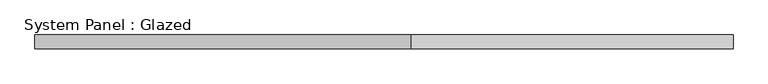
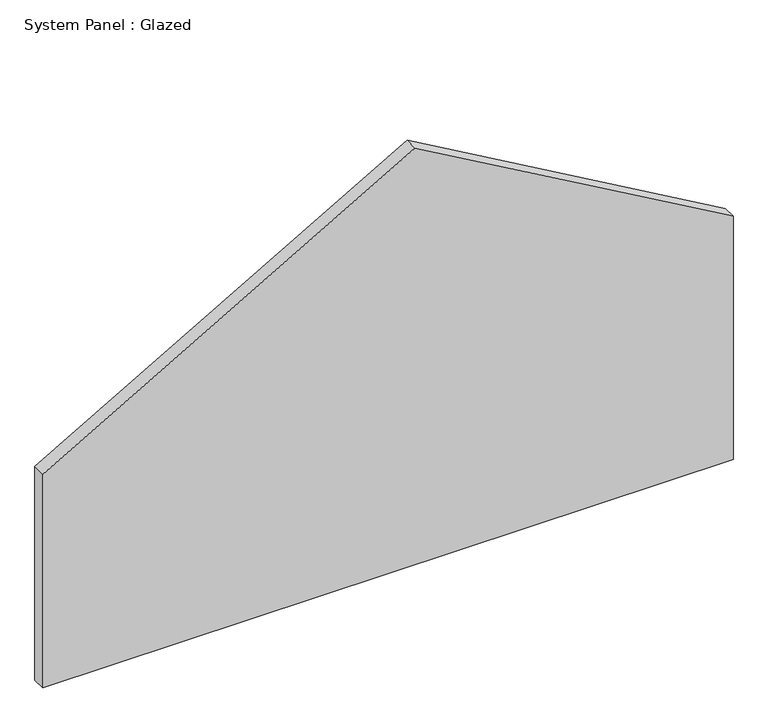
"""IFC4 building model written with IfcOpenShell, lengths in millimetres: plate geometry, System Panel : Glazed."""

from ifc_helpers import new_model, si_unit, frame, origin, place, context, project, spatial, polyline, outline, extrude, source, transform, mapped, element, save


def system_panel_glazed_71429794(model_context):
    return source(origin(), model_context, "Body", "SweptSolid", [
        extrude(outline(polyline([(0.0, -639.2857142), (0.0, 639.2857142), (476.2276186, 639.2857142), (816.4518843, 50.0), (418.4925917, -639.2857142), (0.0, -639.2857142)])), frame((0.0, 24.5, 0.0), z_axis=(0.0, 1.0, 0.0), x_axis=(0.0, 0.0, 1.0)), (0.0, 0.0, 1.0), 25.0),
    ])


if __name__ == "__main__":
    model = new_model("IFC4")
    model_context = context("Model", 3, world=origin())
    ifc_project = project(units=[si_unit("LENGTHUNIT", "METRE", prefix="MILLI")], contexts=[model_context])
    site = spatial("IfcSite", under=ifc_project)
    building = spatial("IfcBuilding", under=site)
    placement = place(None, origin())
    system_panel_glazed_shape = system_panel_glazed_71429794(model_context)
    element("IfcPlate", 1, ObjectType="System Panel : Glazed", at=placement, inside=building, context=model_context, shape_type="MappedRepresentation", body=[
        mapped(system_panel_glazed_shape, transform((0.0, 0.0, 0.0), x_axis=(1.0, 0.0, 0.0), y_axis=(0.0, 1.0, 0.0), z_axis=(0.0, 0.0, 1.0))),
    ])
    save(model, "model.ifc")

# Revit data of these elements
# Type "System Panel : Glazed"
#   Construction Type Id = "GSP4R"
#   Analytic Construction = "1/8 in Pilkington single glazing"
#   Visual Light Transmittance = 0.9
#   Solar Heat Gain Coefficient = 0.86
#   Heat Transfer Coefficient (U) = 6.7069 W/(m²·K)
#   Define Thermal Properties by = 1
# Element 1 (IfcPlate, "System Panel : Glazed")
#   Materials on its faces: "Glass"
# Materials
#   "Glass": class "Glass", colour RGB 0 128 192, transparency 0.75, Description = "Soda Lime Glass", Cost = 0
